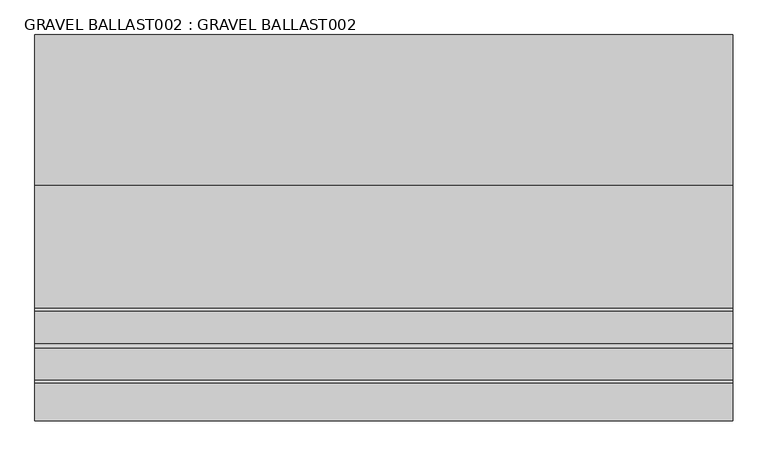
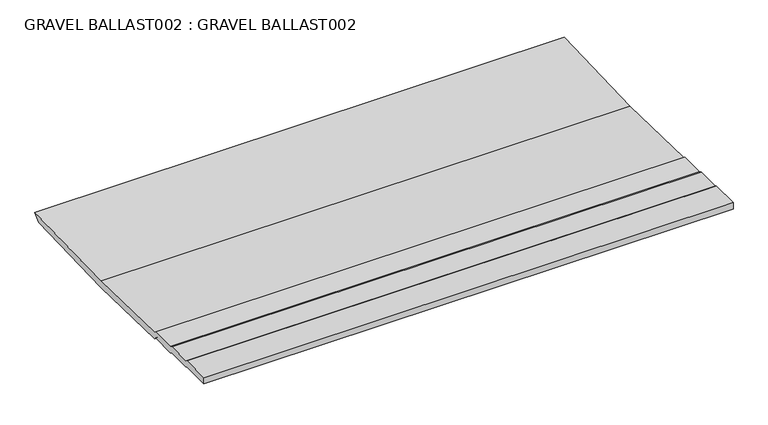
"""IFC4 building model written with IfcOpenShell, lengths in millimetres: proxy geometry, GRAVEL BALLAST002 : GRAVEL BALLAST002."""

from ifc_helpers import new_model, si_unit, frame, origin, place, context, project, spatial, polyline, outline, extrude, source, transform, mapped, element, save


def gravel_ballast002_gravel_ballast002_c19f6b3d(model_context):
    return source(origin(), model_context, "Body", "SweptSolid", [
        extrude(outline(polyline([(-5440.365918, 40253.79375), (-5549.8654297, 40253.79375), (-5549.8654297, 40278.5320313), (-5440.365918, 40278.5320313), (-5431.6554687, 40274.2507813), (-5341.0685547, 40274.2507813), (-5328.2239153, 40268.5233193), (-5234.272168, 40270.16875), (-5225.9987305, 40262.7585938), (-4873.4420898, 40254.5398438), (-4442.8393555, 40268.1982422), (-4468.0649414, 40242.9726562), (-4873.4420898, 40229.8015625), (-5225.9987305, 40238.0203125), (-5234.272168, 40245.4304687), (-5328.2239153, 40243.785038), (-5341.0685547, 40249.5125), (-5431.6554687, 40249.5125), (-5440.365918, 40253.79375)])), frame((12382.7678845, 0.0, 0.0), z_axis=(1.0, 0.0, 0.0), x_axis=(0.0, 1.0, 0.0)), (0.0, 0.0, 1.0), 2000.0),
    ])


if __name__ == "__main__":
    model = new_model("IFC4")
    model_context = context("Model", 3, world=origin())
    ifc_project = project(units=[si_unit("LENGTHUNIT", "METRE", prefix="MILLI")], contexts=[model_context])
    site = spatial("IfcSite", under=ifc_project)
    building = spatial("IfcBuilding", under=site)
    placement = place(None, origin())
    gravel_ballast002_gravel_ballast002_shape = gravel_ballast002_gravel_ballast002_c19f6b3d(model_context)
    element("IfcBuildingElementProxy", 1, Name="GRAVEL BALLAST002 : GRAVEL BALLAST002", ObjectType="GRAVEL BALLAST002 : GRAVEL BALLAST002", at=placement, inside=building, context=model_context, shape_type="MappedRepresentation", body=[
        mapped(gravel_ballast002_gravel_ballast002_shape, transform((0.0, 0.0, 0.0), x_axis=(1.0, 0.0, 0.0), y_axis=(0.0, 1.0, 0.0), z_axis=(0.0, 0.0, 1.0))),
    ])
    save(model, "model.ifc")

# Revit data of these elements
# Type "GRAVEL BALLAST002 : GRAVEL BALLAST002"
#   NameOverride = "GRAVEL BALLAST002"
# Element 1 (IfcBuildingElementProxy, "GRAVEL BALLAST002 : GRAVEL BALLAST002")
#   Materials on its faces: "GRAVEL BALLAST"
# Materials
#   "GRAVEL BALLAST": class "Unassigned", colour RGB 128 128 128, transparency 0, Cost = 0
